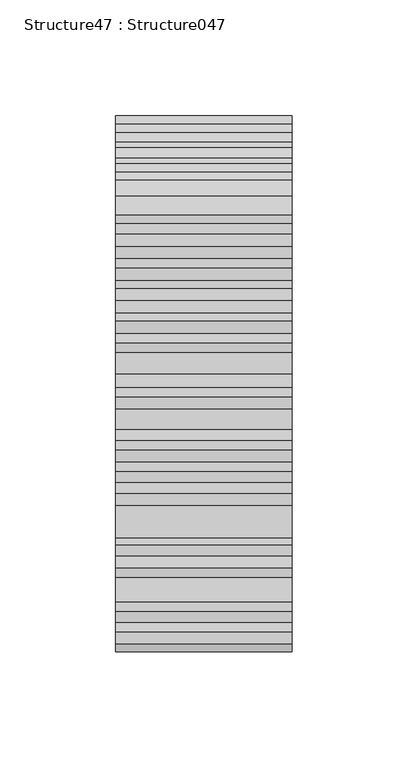
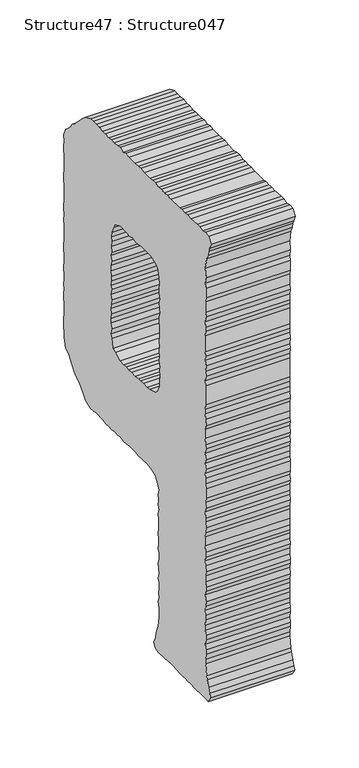
"""IFC4 building model written with IfcOpenShell, lengths in millimetres: proxy geometry, Structure47 : Structure047."""

from ifc_helpers import new_model, si_unit, frame, origin, place, context, project, spatial, polyline, outline, extrude, source, transform, mapped, element, save


def structure47_structure047_346fd536(model_context):
    return source(origin(), model_context, "Body", "SweptSolid", [
        extrude(outline(polyline([(252146.4119108, 3996.390138), (252151.6798274, 3997.5486624), (252155.7876149, 3996.9645864), (252161.6556535, 3996.390138), (252171.0233346, 3996.390138), (252175.1230991, 3997.5486624), (252179.2228635, 3996.390138), (252184.5068261, 3997.5486624), (252188.0160962, 3996.9645864), (252193.2824081, 3996.9645864), (252198.5663707, 3996.390138), (252202.0756408, 3996.390138), (252207.3596034, 3996.9645864), (252211.4433218, 3996.9645864), (252216.7272844, 3997.5486624), (252222.0016194, 3996.9645864), (252226.6854599, 3996.9645864), (252230.19473, 3997.5486624), (252238.4038866, 3994.0233463), (252245.428845, 3987.5792547), (252248.9461381, 3983.4794902), (252252.4634311, 3980.5623192), (252254.8141767, 3977.6194746), (252259.4964126, 3974.1214368), (252261.8391352, 3970.5768654), (252265.9388997, 3966.5043792), (252269.4577974, 3963.5615346), (252272.9734858, 3955.9348494), (252271.7973107, 3950.6765605), (252272.9734858, 3945.4182716), (252272.9734858, 3941.8753048), (252271.7973107, 3936.6186205), (252271.7973107, 3923.1319197), (252272.9734858, 3918.4480792), (252272.9734858, 3912.5896682), (252271.7973107, 3908.46423), (252272.3894098, 3904.3901392), (252271.7973107, 3899.7046941), (252272.3894098, 3893.822214), (252272.9734858, 3889.7208449), (252272.9734858, 3885.0626781), (252272.3894098, 3880.3627915), (252272.9734858, 3874.5043805), (252272.3894098, 3869.8189354), (252271.7973107, 3865.7015202), (252271.7973107, 3856.3161885), (252272.9734858, 3851.6612309), (252272.9734858, 3846.3772683), (252271.7973107, 3841.6741725), (252271.7973107, 3838.1761347), (252272.9734858, 3827.6162325), (252272.3894098, 3822.348316), (252271.7973107, 3818.8310229), (252272.9734858, 3812.9726119), (252272.3894098, 3808.8888934), (252272.9734858, 3804.1890069), (252272.9734858, 3799.5051664), (252272.3894098, 3795.4037973), (252271.7973107, 3790.1294623), (252272.3894098, 3784.8438951), (252272.9734858, 3780.1616592), (252272.9734858, 3771.9605256), (252271.7973107, 3767.2590344), (252271.7973107, 3762.5848215), (252270.0482918, 3753.2171405), (252265.3564283, 3750.8583719), (252263.0137057, 3747.3587295), (252255.9887472, 3739.1592005), (252253.0459026, 3736.2163558), (252248.3716897, 3733.8736333), (252242.503651, 3726.8566978), (252238.4038866, 3722.1568112), (252230.19473, 3719.2316172), (252226.6854599, 3719.8140887), (252221.419148, 3720.4158154), (252211.4433218, 3720.4158154), (252206.7675043, 3719.2316172), (252202.0756408, 3719.8140887), (252197.3837772, 3719.2316172), (252193.8745072, 3719.8140887), (252188.0160962, 3719.8140887), (252183.9163317, 3720.4158154), (252178.6403921, 3719.2316172), (252175.1230991, 3719.8140887), (252169.2727111, 3720.4158154), (252160.4714554, 3720.4158154), (252155.1955158, 3719.2316172), (252151.1037744, 3719.8140887), (252147.0040099, 3719.8140887), (252142.3121463, 3720.4158154), (252136.4521307, 3719.2316172), (252128.8270501, 3716.8985223), (252126.4939552, 3713.9556777), (252122.9766622, 3706.3289925), (252124.1528373, 3702.229228), (252123.5607382, 3696.3884676), (252124.1528373, 3691.6869765), (252122.9766622, 3687.587212), (252124.1528373, 3683.4858429), (252123.5607382, 3677.6274319), (252123.5607382, 3668.8261762), (252124.1528373, 3664.1423357), (252123.5607382, 3659.4584952), (252123.5607382, 3654.7842823), (252124.1528373, 3649.5003197), (252122.9766622, 3645.9830266), (252122.9766622, 3640.7167147), (252124.1528373, 3636.0408972), (252123.5607382, 3630.7392839), (252122.9766622, 3626.6571701), (252124.1528373, 3621.3732075), (252122.9766622, 3617.8559144), (252122.9766622, 3613.1720739), (252123.5607382, 3607.3393366), (252122.9766622, 3603.7963698), (252124.1528373, 3599.1125293), (252122.9766622, 3593.2541183), (252122.9766622, 3584.4689087), (252124.1528373, 3575.0851816), (252127.0764266, 3569.2524442), (252128.8270501, 3559.8671125), (252131.1777957, 3556.3417965), (252128.8270501, 3551.6675836), (252124.1528373, 3550.4833855), (252114.1850341, 3550.4833855), (252108.9171176, 3551.0658569), (252104.8173531, 3551.6675836), (252101.30006, 3551.6675836), (252090.7578085, 3550.4833855), (252086.6484164, 3550.4833855), (252081.9645759, 3551.0658569), (252077.8567883, 3550.4833855), (252073.1729478, 3551.0658569), (252067.9050313, 3550.4833855), (252063.2131677, 3550.4833855), (252059.6958747, 3551.0658569), (252049.7376992, 3551.0658569), (252045.6363301, 3550.4833855), (252042.1286646, 3556.3417965), (252043.2855845, 3559.8671125), (252045.0538586, 3564.54293), (252047.3869536, 3570.4109687), (252047.9790526, 3573.9266571), (252049.7376992, 3584.4689087), (252049.7376992, 3588.5702778), (252049.1536231, 3593.8285667), (252049.1536231, 3597.9540049), (252050.3201706, 3602.6298224), (252049.1536231, 3607.8961343), (252049.1536231, 3612.0135494), (252050.3201706, 3616.0972679), (252050.3201706, 3620.7971545), (252049.7376992, 3626.6571701), (252049.7376992, 3630.7392839), (252050.3201706, 3635.4407751), (252049.7376992, 3639.5405396), (252049.1536231, 3644.2420307), (252050.3201706, 3650.1004418), (252049.1536231, 3654.1841602), (252049.1536231, 3658.3015753), (252049.7376992, 3662.9854159), (252049.7376992, 3668.8261762), (252049.1536231, 3672.9435914), (252049.7376992, 3678.2018803), (252050.3201706, 3682.8857208), (252049.7376992, 3686.4030139), (252049.7376992, 3691.0868544), (252050.3201706, 3696.9709391), (252050.3201706, 3705.7545441), (252049.7376992, 3709.8559132), (252049.1536231, 3715.1302482), (252049.7376992, 3720.4158154), (252049.7376992, 3723.9154578), (252050.3201706, 3729.7738688), (252049.1536231, 3733.8736333), (252049.7376992, 3739.1592005), (252049.1536231, 3743.2332913), (252049.1536231, 3752.6170184), (252049.7376992, 3756.7440611), (252049.7376992, 3762.0023501), (252050.3201706, 3766.684586), (252049.1536231, 3771.3860772), (252050.3201706, 3776.0618947), (252049.1536231, 3780.1616592), (252050.3201706, 3786.0280932), (252049.1536231, 3790.7039107), (252049.7376992, 3794.2292268), (252050.3201706, 3800.0876378), (252050.3201706, 3808.8888934), (252049.1536231, 3812.9726119), (252049.7376992, 3818.8310229), (252050.3201706, 3823.5341187), (252050.3201706, 3828.2163546), (252049.7376992, 3832.8921721), (252049.7376992, 3851.0595042), (252050.3201706, 3855.1769193), (252049.1536231, 3860.4432313), (252049.7376992, 3864.5446004), (252049.1536231, 3870.4030114), (252050.3201706, 3875.0772243), (252049.7376992, 3879.1769888), (252050.3201706, 3883.2863809), (252050.3201706, 3898.5301236), (252049.7376992, 3903.2059411), (252049.7376992, 3906.7328618), (252050.3201706, 3912.0071968), (252049.1536231, 3917.2735087), (252049.7376992, 3921.3748778), (252049.7376992, 3931.3346579), (252049.1536231, 3935.4328178), (252049.1536231, 3944.8165449), (252050.3201706, 3948.917914), (252049.1536231, 3954.7506513), (252050.3201706, 3962.9774586), (252047.9790526, 3973.5197101), (252046.2284291, 3978.2035506), (252045.0538586, 3982.8793681), (252043.2855845, 3986.4046842), (252041.5365656, 3991.6806238), (252045.0538586, 3996.9645864), (252050.3201706, 3997.5486624), (252054.4215397, 3996.390138), (252059.1134032, 3997.5486624), (252063.2131677, 3997.5486624), (252073.7554193, 3996.390138), (252077.8567883, 3997.5486624), (252083.1407509, 3996.390138), (252087.8149638, 3996.9645864), (252090.7578085, 3996.390138), (252104.8173531, 3996.390138), (252110.083665, 3996.9645864), (252114.7675056, 3996.390138), (252119.4593691, 3996.9645864), (252123.5607382, 3996.390138), (252128.8270501, 3997.5486624), (252132.9364423, 3997.5486624), (252137.6202828, 3996.390138), (252146.4119108, 3996.390138)]), holes=[polyline([(252128.2526017, 3797.1463977), (252137.6202828, 3794.2292268), (252141.7280703, 3793.6451507), (252147.0040099, 3794.2292268), (252151.6798274, 3793.6451507), (252155.1955158, 3793.6451507), (252160.4714554, 3793.0723069), (252165.755418, 3793.6451507), (252170.4312355, 3793.0723069), (252173.9485286, 3793.6451507), (252178.6403921, 3793.0723069), (252183.9163317, 3793.6451507), (252190.9412902, 3797.1463977), (252195.0506823, 3798.9050443), (252196.7997012, 3807.1045732), (252197.9742717, 3810.6298893), (252196.7997012, 3816.4883003), (252197.9742717, 3821.1737455), (252197.9742717, 3825.849563), (252197.3837772, 3830.5574726), (252197.9742717, 3835.2332901), (252197.3837772, 3839.3587282), (252196.7997012, 3844.0345457), (252197.9742717, 3848.7167816), (252196.7997012, 3854.0007442), (252197.9742717, 3857.5019912), (252197.3837772, 3862.2018778), (252197.3837772, 3866.3032469), (252197.9742717, 3870.9790644), (252197.9742717, 3876.263027), (252196.7997012, 3880.9452629), (252197.9742717, 3886.2051565), (252196.7997012, 3889.7208449), (252197.3837772, 3895.0048075), (252196.7997012, 3900.2887701), (252197.3837772, 3904.3901392), (252196.7997012, 3909.0627475), (252193.8745072, 3915.5068392), (252192.1254883, 3919.0321552), (252184.5068261, 3921.9733953), (252175.1230991, 3921.9733953), (252169.2727111, 3921.3748778), (252165.163319, 3922.5494483), (252159.888984, 3921.3748778), (252156.3716909, 3921.9733953), (252151.6798274, 3922.5494483), (252137.0362067, 3922.5494483), (252128.2526017, 3919.6066036), (252125.3193847, 3916.0909152), (252123.5607382, 3909.0627475), (252122.9766622, 3904.3901392), (252123.5607382, 3899.7046941), (252123.5607382, 3894.4030808), (252122.3941907, 3889.7208449), (252123.5607382, 3886.2051565), (252122.9766622, 3880.3627915), (252122.3941907, 3876.263027), (252123.5607382, 3871.5599312), (252123.5607382, 3867.4601667), (252122.9766622, 3862.8036045), (252122.9766622, 3853.4198774), (252123.5607382, 3848.1166595), (252122.9766622, 3844.6154125), (252123.5607382, 3839.3587282), (252122.9766622, 3834.0474873), (252123.5607382, 3829.9733965), (252122.3941907, 3824.7167122), (252122.9766622, 3821.1737455), (252122.3941907, 3816.4883003), (252122.9766622, 3810.6298893), (252122.9766622, 3805.9476534), (252125.9018562, 3799.5051664), (252128.2526017, 3797.1463977)])]), frame((-38594.2176606, 0.0, 0.0), z_axis=(1.0, 0.0, 0.0), x_axis=(0.0, 1.0, 0.0)), (0.0, 0.0, 1.0), 76.2),
    ])


if __name__ == "__main__":
    model = new_model("IFC4")
    model_context = context("Model", 3, world=origin())
    ifc_project = project(units=[si_unit("LENGTHUNIT", "METRE", prefix="MILLI")], contexts=[model_context])
    site = spatial("IfcSite", under=ifc_project)
    building = spatial("IfcBuilding", under=site)
    placement = place(None, origin())
    structure47_structure047_shape = structure47_structure047_346fd536(model_context)
    element("IfcBuildingElementProxy", 1, Name="Structure47 : Structure047", ObjectType="Structure47 : Structure047", at=placement, inside=building, context=model_context, shape_type="MappedRepresentation", body=[
        mapped(structure47_structure047_shape, transform((0.0, 0.0, 0.0), x_axis=(1.0, 0.0, 0.0), y_axis=(0.0, 1.0, 0.0), z_axis=(0.0, 0.0, 1.0))),
    ])
    save(model, "model.ifc")

# Revit data of these elements
# Type "Structure47 : Structure047"
#   NameOverride = "Structure047"
# Element 1 (IfcBuildingElementProxy, "Structure47 : Structure047")
#   Materials on its faces: "BRUSHED ALUM. LETTERING"
# Materials
#   "BRUSHED ALUM. LETTERING": class "Unassigned", colour RGB 169 181 186, transparency 0, Cost = 0
